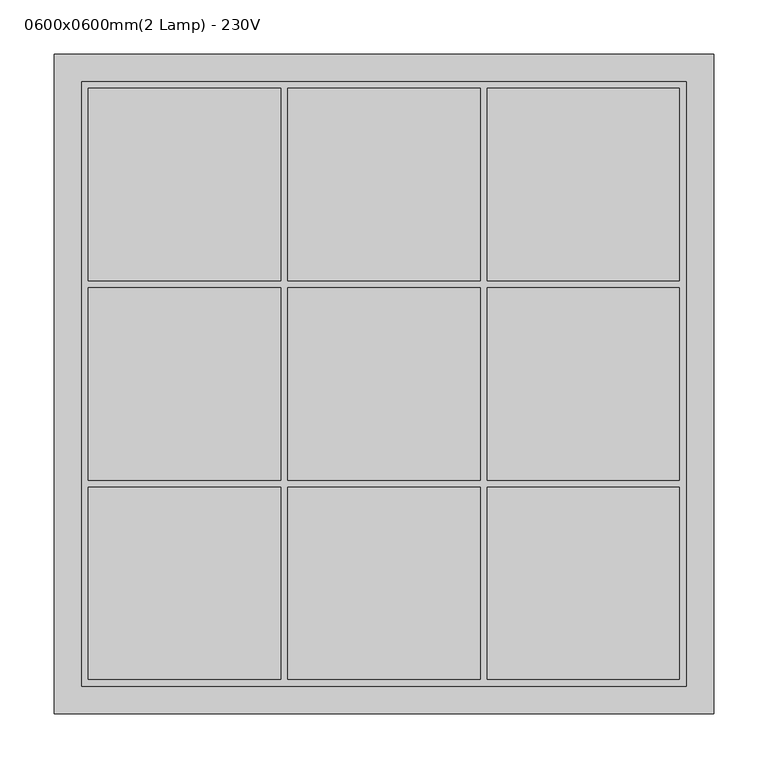
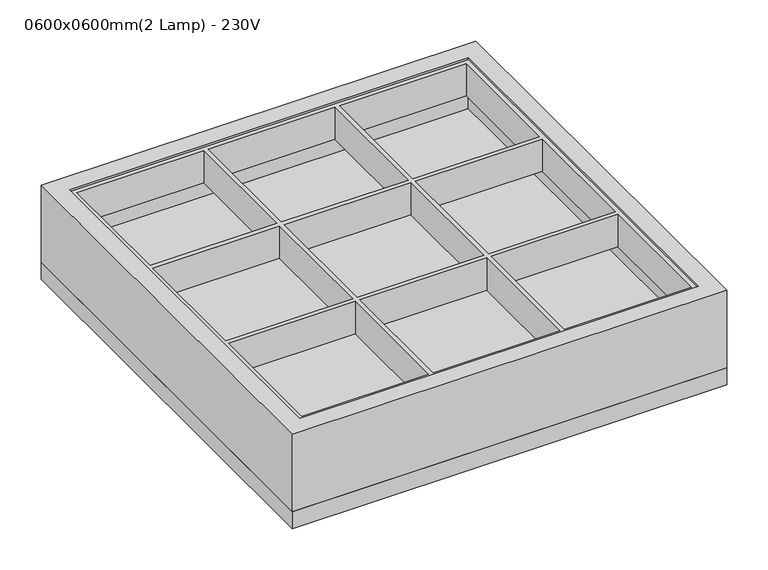
"""IFC4 building model written with IfcOpenShell, lengths in millimetres: light fixture geometry, Coffer Light - Parabolic Square : 0600x0600mm(2 Lamp) - 230V."""

from ifc_helpers import new_model, si_unit, frame, origin, place, context, project, spatial, polyline, outline, extrude, source, transform, mapped, element, save


def light_fixture_0600x0600mm_2_lamp_230v_801c9e30(model_context):
    return source(origin(), model_context, "Body", "SweptSolid", [
        extrude(outline(polyline([(279.4, -25.4), (279.4, -584.2), (-279.4, -584.2), (-279.4, -25.4), (279.4, -25.4)]), holes=[polyline([(95.25, -400.05), (95.25, -577.85), (273.05, -577.85), (273.05, -400.05), (95.25, -400.05)]), polyline([(-273.05, -400.05), (-273.05, -577.85), (-95.25, -577.85), (-95.25, -400.05), (-273.05, -400.05)]), polyline([(88.9, -577.85), (88.9, -400.05), (-88.9, -400.05), (-88.9, -577.85), (88.9, -577.85)]), polyline([(-273.05, -31.75), (-273.05, -209.55), (-95.25, -209.55), (-95.25, -31.75), (-273.05, -31.75)]), polyline([(-88.9, -31.75), (-88.9, -209.55), (88.9, -209.55), (88.9, -31.75), (-88.9, -31.75)]), polyline([(95.25, -31.75), (95.25, -209.55), (273.05, -209.55), (273.05, -31.75), (95.25, -31.75)]), polyline([(95.25, -215.9), (95.25, -393.7), (273.05, -393.7), (273.05, -215.9), (95.25, -215.9)]), polyline([(-88.9, -215.9), (-88.9, -393.7), (88.9, -393.7), (88.9, -215.9), (-88.9, -215.9)]), polyline([(-273.05, -215.9), (-273.05, -393.7), (-95.25, -393.7), (-95.25, -215.9), (-273.05, -215.9)])]), frame((0.0, 0.0, -50.8), z_axis=(0.0, 0.0, 1.0), x_axis=(1.0, 0.0, 0.0)), (0.0, 0.0, 1.0), 47.625),
        extrude(outline(polyline([(279.4, -25.4), (279.4, -584.2), (-279.4, -584.2), (-279.4, -25.4), (279.4, -25.4)])), frame((0.0, 0.0, -82.55), z_axis=(0.0, 0.0, 1.0), x_axis=(1.0, 0.0, 0.0)), (0.0, 0.0, 1.0), 6.35),
        extrude(outline(polyline([(-304.8, -609.6), (-304.8, 0.0), (304.8, 0.0), (304.8, -609.6), (-304.8, -609.6)]), holes=[polyline([(279.4, -25.4), (-279.4, -25.4), (-279.4, -584.2), (279.4, -584.2), (279.4, -25.4)])]), frame((0.0, 0.0, -114.3), z_axis=(0.0, 0.0, 1.0), x_axis=(1.0, 0.0, 0.0)), (0.0, 0.0, 1.0), 114.3),
        extrude(outline(polyline([(304.8, 0.0), (304.8, -609.6), (-304.8, -609.6), (-304.8, 0.0), (304.8, 0.0)])), frame((0.0, 0.0, -139.7), z_axis=(0.0, 0.0, 1.0), x_axis=(1.0, 0.0, 0.0)), (0.0, 0.0, 1.0), 25.4),
    ])


if __name__ == "__main__":
    model = new_model("IFC4")
    model_context = context("Model", 3, world=origin())
    ifc_project = project(units=[si_unit("LENGTHUNIT", "METRE", prefix="MILLI")], contexts=[model_context])
    site = spatial("IfcSite", under=ifc_project)
    building = spatial("IfcBuilding", under=site)
    placement = place(None, origin())
    light_fixture_0600x0600mm_2_lamp_230v_shape = light_fixture_0600x0600mm_2_lamp_230v_801c9e30(model_context)
    element("IfcLightFixture", 1, ObjectType="Coffer Light - Parabolic Square : 0600x0600mm(2 Lamp) - 230V", at=placement, inside=building, context=model_context, shape_type="MappedRepresentation", body=[
        mapped(light_fixture_0600x0600mm_2_lamp_230v_shape, transform((0.0, 0.0, 0.0), x_axis=(1.0, 0.0, 0.0), y_axis=(0.0, 1.0, 0.0), z_axis=(0.0, 0.0, 1.0))),
    ])
    save(model, "model.ifc")

# Revit data of these elements
# Type "Coffer Light - Parabolic Square : 0600x0600mm(2 Lamp) - 230V"
#   Type Mark = "Coffer Light - Parabolic Square"
#   Classification.OmniClass.23.Number = "23-35 47 11 21 17"
#   Classification.OmniClass.23.Description = "Buried Uplights"
#   COBie.Type.CreatedBy = "info@mma.ie"
#   COBie.Type.CreatedOn = "2017-07-25T10:15:16"
#   COBie.Type.Name = "Coffer Light - Parabolic Square"
#   COBie.Type.Category = "23-35 47 11 21 17 : Buried Uplights"
#   COBie.Type.Description = "Coffer Light - Parabolic Square_0600x0600mm(2 Lamp) - 230V"
#   COBie.Type.AssetType = "Fixed"
#   COBie.Type.Manufacturer = ""
#   COBie.Type.ModelNumber = ""
#   Photometric Web File = "2x22T12.ies"
#   Lamp = "T-12"
#   Keynote = "26 51 13.C"
#   COBie.Type.ReplacementCost = 0
#   Wattage = 40 W
#   built-in parameter 1150110 = 1 (stored number, unit not read)
#   built-in parameter 1150109 = 1 (stored number, unit not read)
#   built-in parameter 1150113 = 1 (stored number, unit not read)
#   Tilt Angle = -90.00°
#   Lumens = 2600 lm
#   built-in parameter 1114217 = 0.88 (stored number, unit not read)
#   built-in parameter 1150115 = 1 (stored number, unit not read)
#   built-in parameter 1150105 = 206.901 (stored number, unit not read)
#   built-in parameter 1150112 = 1 (stored number, unit not read)
#   built-in parameter 1150114 = 1 (stored number, unit not read)
#   built-in parameter 1150107 = 4230 (stored number, unit not read)
#   built-in parameter 1150106 = 2.06901 (stored number, unit not read)
#   Emit from Rectangle Width = 559.6 mm
#   Emit from Rectangle Length = 559.6 mm
#   built-in parameter 1150104 = 6.0387 (stored number, unit not read)
#   Default Elevation = 1200 mm
#   Coffer.L- Width = 609.6 mm
#   Coffer.L- Length = 609.6 mm
#   Ballast Voltage = 230 V
#   built-in parameter 1114218 = 0.88 (stored number, unit not read)
#   built-in parameter 1150133 = 10 (stored number, unit not read)
#   Apparent Load = 40 VA
#   COBie.Type = yes
#   built-in parameter 1150134 = 8
#   built-in parameter 1150137 = 1
#   Color Filter = 16777215
#   built-in parameter 1140040 [instance default] = 1
#   Ballast Number of Poles = 1
#   Load Classification = Lighting - Dwelling Unit
#   Light Box Material = Metal - Chrome
#   Grid Material = Metal - Paint Finish - Dark Grey, Matt
#   Diffuser Material = Glass - White, High Luminance
#   Coffer.L- Material = Metal - Chrome
#   Emit Shape Visible in Rendering = no
#   Dimming Lamp Color Temperature Shift = (empty or 0)
#   Assembly Code = ""
# Element 1 (IfcLightFixture, "Coffer Light - Parabolic Square : 0600x0600mm(2 Lamp) - 230V")
#   Materials on its faces: "Metal - Paint Finish - Dark Grey, Matt", "Metal - Chrome", "Glass - White, High Luminance"
# Materials
#   "Metal - Chrome": class "Metal", colour RGB 17 17 17, transparency 0, Comments = "Rendering appearance not upgraded "
#   "Metal - Paint Finish - Dark Grey, Matt": class "Paint", colour RGB 98 98 98, transparency 0
#   "Glass - White, High Luminance": class "Glass", colour RGB 249 250 249, transparency 0.8
